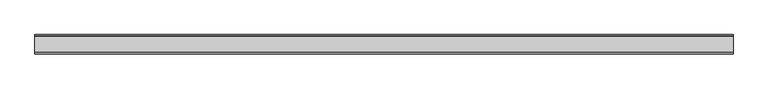
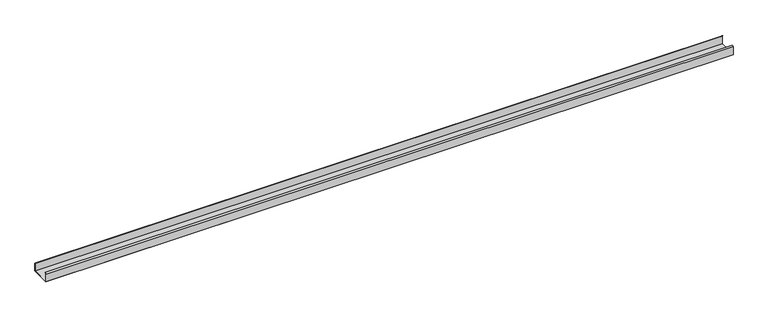
"""IFC4 building model written with IfcOpenShell, lengths in millimetres: proxy geometry, Generic Models 7:Generic Models 1:1:Generic Models 1:1 : Generic Models 7:Generic Models 1:337419:2 : Generic Models 7:Generic Models 1:1:Generic Models 1:1 : Generic Models 7:Generic Models 1:337419:306201."""

from ifc_helpers import new_model, si_unit, frame, origin, place, context, project, spatial, polyline, outline, extrude, source, transform, mapped, element, save


def generic_models_f69d2429(model_context):
    return source(origin(), model_context, "Body", "SweptSolid", [
        extrude(outline(polyline([(-578797.4913841, 3675.0625), (-579000.6913841, 3675.0625), (-579000.6913841, 3763.9625), (-578986.0982375, 3776.207604), (-578984.3124931, 3774.0794367), (-578997.9132591, 3762.667039), (-578997.9132591, 3677.840625), (-578800.2695091, 3677.840625), (-578800.2695091, 3762.667039), (-578813.8702751, 3774.0794367), (-578812.0845307, 3776.207604), (-578797.4913841, 3763.9625), (-578797.4913841, 3675.0625)])), frame((565582.1867239, 0.0, 0.0), z_axis=(1.0, 0.0, 0.0), x_axis=(0.0, 1.0, 0.0)), (0.0, 0.0, 1.0), 7315.2),
    ])


if __name__ == "__main__":
    model = new_model("IFC4")
    model_context = context("Model", 3, world=origin())
    ifc_project = project(units=[si_unit("LENGTHUNIT", "METRE", prefix="MILLI")], contexts=[model_context])
    site = spatial("IfcSite", under=ifc_project)
    building = spatial("IfcBuilding", under=site)
    placement = place(None, origin())
    generic_models_shape = generic_models_f69d2429(model_context)
    element("IfcBuildingElementProxy", 1, Name="Generic Models 7:Generic Models 1:1:Generic Models 1:1 : Generic Models 7:Generic Models 1:337419:2 : Generic Models 7:Generic Models 1:1:Generic Models 1:1 : Generic Models 7:Generic Models 1:337419:306201", ObjectType="Generic Models 7:Generic Models 1:1:Generic Models 1:1 : Generic Models 7:Generic Models 1:337419:2 : Generic Models 7:Generic Models 1:1:Generic Models 1:1 : Generic Models 7:Generic Models 1:337419:306201", at=placement, inside=building, context=model_context, shape_type="MappedRepresentation", body=[
        mapped(generic_models_shape, transform((0.0, 0.0, 0.0), x_axis=(1.0, 0.0, 0.0), y_axis=(0.0, 1.0, 0.0), z_axis=(0.0, 0.0, 1.0))),
    ])
    save(model, "model.ifc")

# Revit data of these elements
# Type "Generic Models 7:Generic Models 1:1:Generic Models 1:1 : Generic Models 7:Generic Models 1:337419:2 : Generic Models 7:Generic Models 1:1:Generic Models 1:1 : Generic Models 7:Generic Models 1:337419:306201"
#   NameOverride = "Generic Models 7:Generic Models 1:1:Generic Models 1:1 : Generic Models 7:Generic Models 1:337419:306201"
#   ObjectTypeOverride = "Generic Models 1:1 : Generic Models 7:Generic Models 1:337419"
#   Reference = "Generic Models 1"
#   Tag = "306201"
# Element 1 (IfcBuildingElementProxy, "Generic Models 7:Generic Models 1:1:Generic Models 1:1 : Generic Models 7:Generic Models 1:337419:2 : Generic Models 7:Generic Models 1:1:Generic Models 1:1 : Generic Models 7:Generic Models 1:337419:306201")
#   Materials on its faces: "'ZEE' SECTION (8.0x3.5Z - SEE STRUCT. DWGS)"
# Materials
#   "'ZEE' SECTION (8.0x3.5Z - SEE STRUCT. DWGS)": class "Unassigned", colour RGB 210 209 208, transparency 0, Keynote = "M05121300.02", Cost = 0
